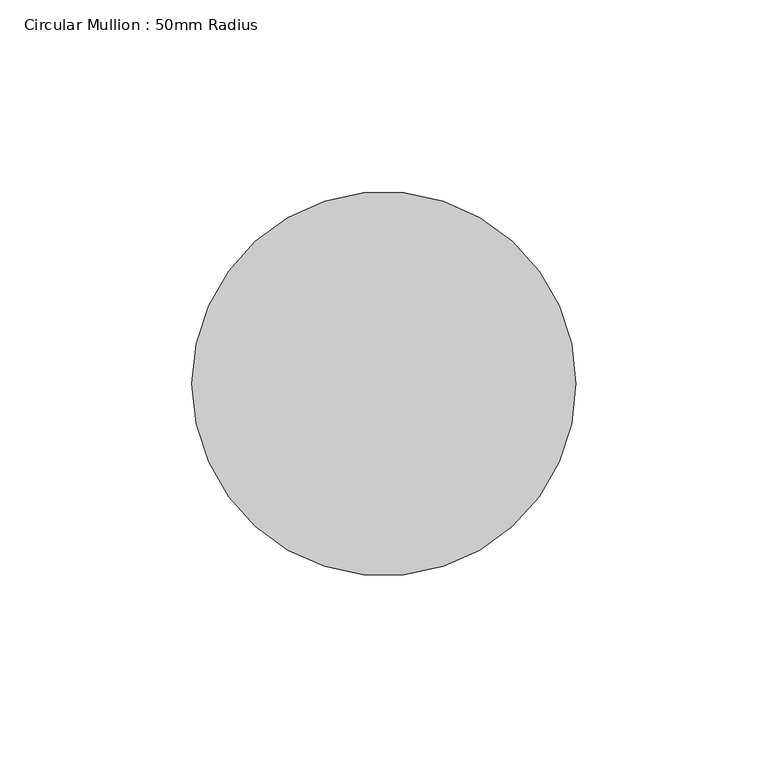
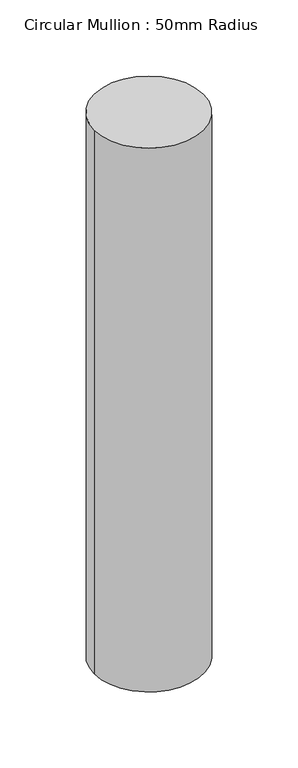
"""IFC4 building model written with IfcOpenShell, lengths in millimetres: member geometry, Circular Mullion : 50mm Radius."""

from ifc_helpers import new_model, si_unit, point, frame, origin, origin_2d, place, context, project, spatial, circle_curve, trimmed, segment, composite_curve, outline, extrude, source, transform, mapped, element, save


def circular_mullion_50mm_radius_2f33ace3(model_context):
    return source(origin(), model_context, "Body", "SweptSolid", [
        extrude(outline(composite_curve([segment(trimmed(circle_curve(origin_2d(), 50.0), [point((50.0, 0.0))], [point((-50.0, 0.0))], False, "CARTESIAN"), True, "CONTINUOUS"), segment(trimmed(circle_curve(origin_2d(), 50.0), [point((-50.0, 0.0))], [point((50.0, 0.0))], False, "CARTESIAN"), True, "CONTINUOUS")], self_intersect=False)), frame((0.0, 0.0, -527.8039477), z_axis=(0.0, 0.0, 1.0), x_axis=(1.0, 0.0, 0.0)), (0.0, 0.0, 1.0), 527.8039477),
    ])


if __name__ == "__main__":
    model = new_model("IFC4")
    model_context = context("Model", 3, world=origin())
    ifc_project = project(units=[si_unit("LENGTHUNIT", "METRE", prefix="MILLI")], contexts=[model_context])
    site = spatial("IfcSite", under=ifc_project)
    building = spatial("IfcBuilding", under=site)
    placement = place(None, origin())
    circular_mullion_50mm_radius_shape = circular_mullion_50mm_radius_2f33ace3(model_context)
    element("IfcMember", 1, ObjectType="Circular Mullion : 50mm Radius", at=placement, inside=building, context=model_context, shape_type="MappedRepresentation", body=[
        mapped(circular_mullion_50mm_radius_shape, transform((0.0, 0.0, 0.0), x_axis=(1.0, 0.0, 0.0), y_axis=(0.0, 1.0, 0.0), z_axis=(0.0, 0.0, 1.0))),
    ])
    save(model, "model.ifc")

# Revit data of these elements
# Type "Circular Mullion : 50mm Radius"
#   built-in parameter 1007350 = 0.164042 (stored number, unit not read)
# Element 1 (IfcMember, "Circular Mullion : 50mm Radius")
#   Materials on its faces: "Aluminium"
# Materials
#   "Aluminium": class "Metal", colour RGB 247 247 247, transparency 0, Description = "Aluminium 6061", Cost = 0
